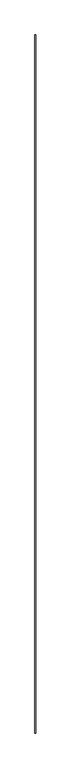
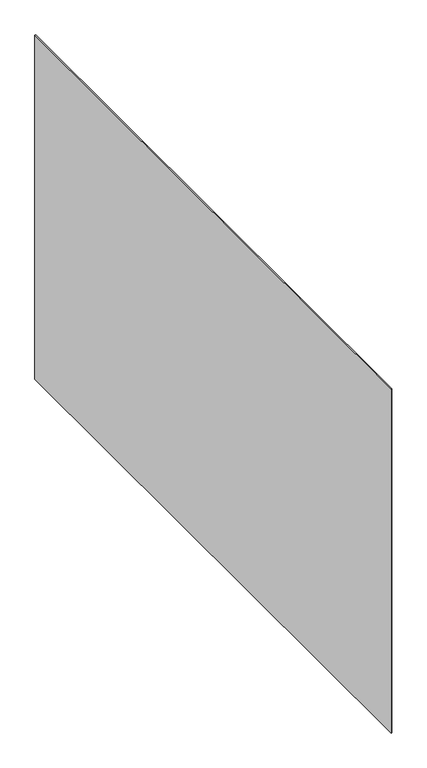
"""IFC4 building model written with IfcOpenShell, lengths in millimetres: proxy geometry, Inner panel:Inner panel:1:Inner panel:1 : Inner panel:Inner panel:300324:300043:Inner panel:1:Inner panel:1 : Inner panel:Inner panel:300324:300043 : Inner panel:Inner panel:1:Inner panel:1 : Inner panel:Inner panel:300324:300043:42 : Inner panel:Inner panel:1:Inner panel:1 : Inner panel:Inner panel:300324:300043:Inner panel:1:Inner panel:1 : Inner panel:Inner panel:300324:300043 : Inner panel:Inner panel:1:Inner panel:1 : Inner panel:Inner panel:300324:300043:300031."""

from ifc_helpers import new_model, si_unit, origin, origin_with_axes, place, context, project, spatial, polyline, outline, extrude, source, transform, mapped, element, save


def generic_models_7dbfeb11(model_context):
    return source(origin(), model_context, "Body", "SweptSolid", [
        extrude(outline(polyline([(667547.3117239, -568256.7847125), (667560.0117239, -568256.7847125), (667560.0117239, -578718.1163841), (667547.3117239, -578718.1163841), (667547.3117239, -568256.7847125)])), origin_with_axes(), (0.0, 0.0, 1.0), 6165.85),
    ])


if __name__ == "__main__":
    model = new_model("IFC4")
    model_context = context("Model", 3, world=origin())
    ifc_project = project(units=[si_unit("LENGTHUNIT", "METRE", prefix="MILLI")], contexts=[model_context])
    site = spatial("IfcSite", under=ifc_project)
    building = spatial("IfcBuilding", under=site)
    placement = place(None, origin())
    generic_models_shape = generic_models_7dbfeb11(model_context)
    element("IfcBuildingElementProxy", 1, Name="Inner panel:Inner panel:1:Inner panel:1 : Inner panel:Inner panel:300324:300043:Inner panel:1:Inner panel:1 : Inner panel:Inner panel:300324:300043 : Inner panel:Inner panel:1:Inner panel:1 : Inner panel:Inner panel:300324:300043:42 : Inner panel:Inner panel:1:Inner panel:1 : Inner panel:Inner panel:300324:300043:Inner panel:1:Inner panel:1 : Inner panel:Inner panel:300324:300043 : Inner panel:Inner panel:1:Inner panel:1 : Inner panel:Inner panel:300324:300043:300031", ObjectType="Inner panel:Inner panel:1:Inner panel:1 : Inner panel:Inner panel:300324:300043:Inner panel:1:Inner panel:1 : Inner panel:Inner panel:300324:300043 : Inner panel:Inner panel:1:Inner panel:1 : Inner panel:Inner panel:300324:300043:42 : Inner panel:Inner panel:1:Inner panel:1 : Inner panel:Inner panel:300324:300043:Inner panel:1:Inner panel:1 : Inner panel:Inner panel:300324:300043 : Inner panel:Inner panel:1:Inner panel:1 : Inner panel:Inner panel:300324:300043:300031", at=placement, inside=building, context=model_context, shape_type="MappedRepresentation", body=[
        mapped(generic_models_shape, transform((0.0, 0.0, 0.0), x_axis=(1.0, 0.0, 0.0), y_axis=(0.0, 1.0, 0.0), z_axis=(0.0, 0.0, 1.0))),
    ])
    save(model, "model.ifc")

# Revit data of these elements
# Type "Inner panel:Inner panel:1:Inner panel:1 : Inner panel:Inner panel:300324:300043:Inner panel:1:Inner panel:1 : Inner panel:Inner panel:300324:300043 : Inner panel:Inner panel:1:Inner panel:1 : Inner panel:Inner panel:300324:300043:42 : Inner panel:Inner panel:1:Inner panel:1 : Inner panel:Inner panel:300324:300043:Inner panel:1:Inner panel:1 : Inner panel:Inner panel:300324:300043 : Inner panel:Inner panel:1:Inner panel:1 : Inner panel:Inner panel:300324:300043:300031"
#   NameOverride = "Inner panel:Inner panel:1:Inner panel:1 : Inner panel:Inner panel:300324:300043:Inner panel:1:Inner panel:1 : Inner panel:Inner panel:300324:300043 : Inner panel:Inner panel:1:Inner panel:1 : Inner panel:Inner panel:300324:300043:300031"
#   ObjectTypeOverride = "Inner panel:1:Inner panel:1 : Inner panel:Inner panel:300324:300043 : Inner panel:Inner panel:1:Inner panel:1 : Inner panel:Inner panel:300324:300043"
#   Reference = "Inner panel"
#   Tag = "300031"
# Element 1 (IfcBuildingElementProxy, "Inner panel:Inner panel:1:Inner panel:1 : Inner panel:Inner panel:300324:300043:Inner panel:1:Inner panel:1 : Inner panel:Inner panel:300324:300043 : Inner panel:Inner panel:1:Inner panel:1 : Inner panel:Inner panel:300324:300043:42 : Inner panel:Inner panel:1:Inner panel:1 : Inner panel:Inner panel:300324:300043:Inner panel:1:Inner panel:1 : Inner panel:Inner panel:300324:300043 : Inner panel:Inner panel:1:Inner panel:1 : Inner panel:Inner panel:300324:300043:300031")
#   Materials on its faces: "1/2\" FIBERGLASS MAT GYPSUM PANELS"
# Materials
#   "1/2\" FIBERGLASS MAT GYPSUM PANELS": class "Generic", colour RGB 171 170 168, transparency 0, Description = "Gypsum Wall Board", Cost = 0
